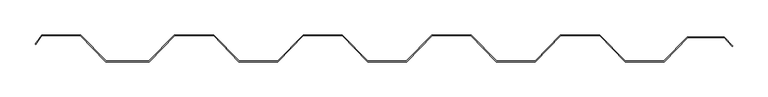
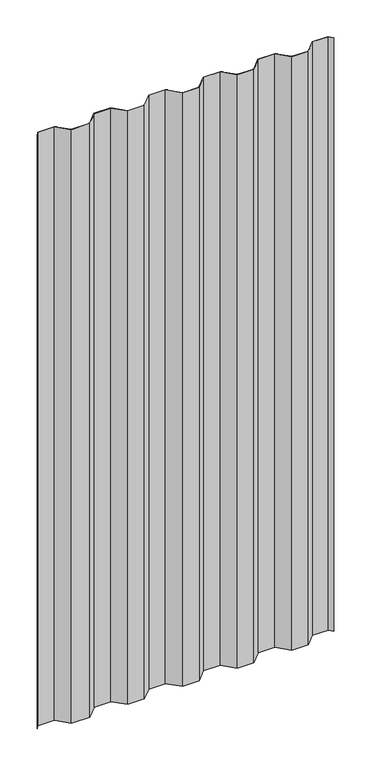
"""IFC4 building model written with IfcOpenShell, lengths in millimetres: proxy geometry, Generic Models 2:Generic Models 2:310765:Generic Models 2:310765 : Generic Models 2:Generic Models 2:310765:56 : Generic Models 2:Generic Models 2:310765:Generic Models 2:310765 : Generic Models 2:Generic Models 2:310765:300385."""

from ifc_helpers import new_model, si_unit, frame, origin, place, context, project, spatial, polyline, outline, extrude, source, transform, mapped, element, save


def generic_models_67275068(model_context):
    return source(origin(), model_context, "Body", "SweptSolid", [
        extrude(outline(polyline([(570516.8090826, -578743.0895469), (570528.6648289, -578756.1976179), (570528.1028571, -578756.7595897), (570516.4567453, -578743.8832969), (570464.5503913, -578743.8832969), (570430.9184065, -578778.4413841), (570375.7388466, -578778.4413841), (570339.5766549, -578741.1351341), (570284.2015293, -578741.1351341), (570248.0393377, -578778.4413841), (570192.8588466, -578778.4413841), (570156.6966549, -578741.1351341), (570101.3215293, -578741.1351341), (570065.1593377, -578778.4413841), (570009.9788466, -578778.4413841), (569973.8166549, -578741.1351341), (569918.4415293, -578741.1351341), (569882.2793377, -578778.4413841), (569827.0988466, -578778.4413841), (569790.9366549, -578741.1351341), (569735.5615293, -578741.1351341), (569699.3993377, -578778.4413841), (569637.8688466, -578778.4413841), (569601.7066549, -578741.1351341), (569547.1780922, -578741.1351341), (569538.2367239, -578753.9047314), (569537.586522, -578753.4494551), (569546.7648921, -578740.3413841), (569602.0427005, -578740.3413841), (569638.2048921, -578777.6476341), (569699.0632921, -578777.6476341), (569735.2254838, -578740.3413841), (569791.2727005, -578740.3413841), (569827.4348921, -578777.6476341), (569881.9432921, -578777.6476341), (569918.1054838, -578740.3413841), (569974.1527005, -578740.3413841), (570010.3148921, -578777.6476341), (570064.8232921, -578777.6476341), (570100.9854838, -578740.3413841), (570157.0327005, -578740.3413841), (570193.1948921, -578777.6476341), (570247.7032921, -578777.6476341), (570283.8654838, -578740.3413841), (570339.9127005, -578740.3413841), (570376.0748921, -578777.6476341), (570430.5832921, -578777.6476341), (570464.2152769, -578743.0895469), (570516.8090826, -578743.0895469)])), frame((0.0, 0.0, 4033.8810286), z_axis=(0.0, 0.0, 1.0), x_axis=(1.0, 0.0, 0.0)), (0.0, 0.0, 1.0), 2100.2189714),
    ])


if __name__ == "__main__":
    model = new_model("IFC4")
    model_context = context("Model", 3, world=origin())
    ifc_project = project(units=[si_unit("LENGTHUNIT", "METRE", prefix="MILLI")], contexts=[model_context])
    site = spatial("IfcSite", under=ifc_project)
    building = spatial("IfcBuilding", under=site)
    placement = place(None, origin())
    generic_models_shape = generic_models_67275068(model_context)
    element("IfcBuildingElementProxy", 1, Name="Generic Models 2:Generic Models 2:310765:Generic Models 2:310765 : Generic Models 2:Generic Models 2:310765:56 : Generic Models 2:Generic Models 2:310765:Generic Models 2:310765 : Generic Models 2:Generic Models 2:310765:300385", ObjectType="Generic Models 2:Generic Models 2:310765:Generic Models 2:310765 : Generic Models 2:Generic Models 2:310765:56 : Generic Models 2:Generic Models 2:310765:Generic Models 2:310765 : Generic Models 2:Generic Models 2:310765:300385", at=placement, inside=building, context=model_context, shape_type="MappedRepresentation", body=[
        mapped(generic_models_shape, transform((0.0, 0.0, 0.0), x_axis=(1.0, 0.0, 0.0), y_axis=(0.0, 1.0, 0.0), z_axis=(0.0, 0.0, 1.0))),
    ])
    save(model, "model.ifc")

# Revit data of these elements
# Type "Generic Models 2:Generic Models 2:310765:Generic Models 2:310765 : Generic Models 2:Generic Models 2:310765:56 : Generic Models 2:Generic Models 2:310765:Generic Models 2:310765 : Generic Models 2:Generic Models 2:310765:300385"
#   NameOverride = "Generic Models 2:Generic Models 2:310765:Generic Models 2:310765 : Generic Models 2:Generic Models 2:310765:300385"
#   ObjectTypeOverride = "Generic Models 2:310765 : Generic Models 2:Generic Models 2:310765"
#   Reference = "Generic Models 2"
#   Tag = "300385"
# Element 1 (IfcBuildingElementProxy, "Generic Models 2:Generic Models 2:310765:Generic Models 2:310765 : Generic Models 2:Generic Models 2:310765:56 : Generic Models 2:Generic Models 2:310765:Generic Models 2:310765 : Generic Models 2:Generic Models 2:310765:300385")
#   Materials on its faces: "VERTICAL CORRUGATED METAL PANEL - EXPOSED FASTENERS - (MBCI 7.2 PANEL)"
# Materials
#   "VERTICAL CORRUGATED METAL PANEL - EXPOSED FASTENERS - (MBCI 7.2 PANEL)": class "Generic", colour RGB 120 120 120, transparency 0, Cost = 0
